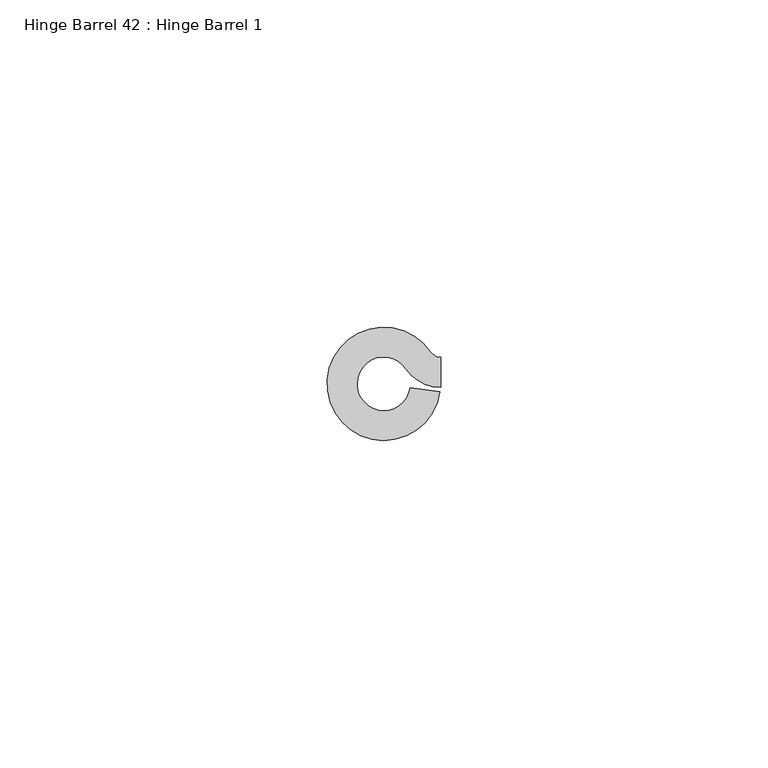
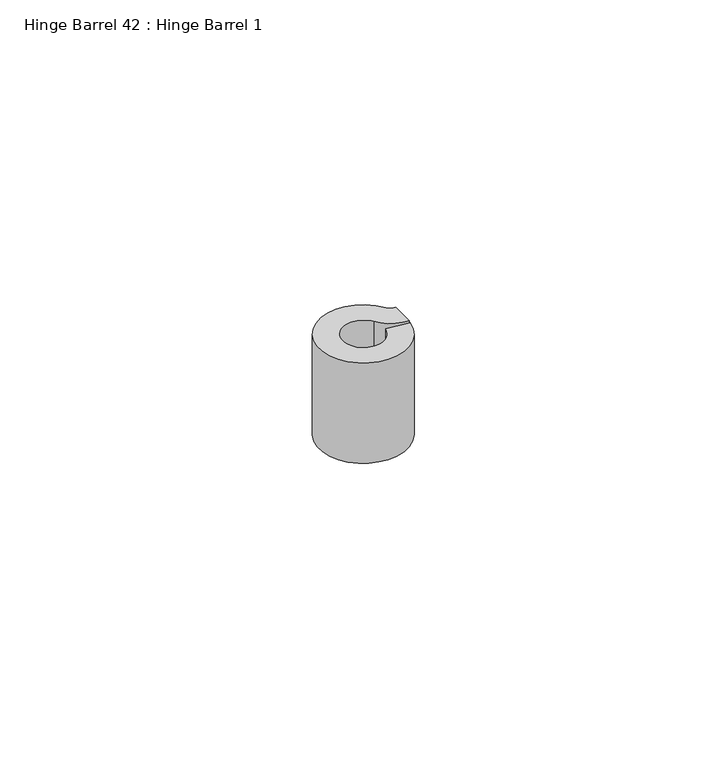
"""IFC4 building model written with IfcOpenShell, lengths in millimetres: proxy geometry, Hinge Barrel 42 : Hinge Barrel 1."""

from ifc_helpers import new_model, si_unit, point, frame, frame_2d, origin, place, context, project, spatial, polyline, circle_curve, trimmed, segment, composite_curve, outline, extrude, source, transform, mapped, element, save


def hinge_barrel_42_hinge_barrel_1_1e33f8db(model_context):
    return source(origin(), model_context, "Body", "SweptSolid", [
        extrude(outline(composite_curve([segment(trimmed(circle_curve(frame_2d((587319.1320739, -534100.7049841)), 4.0894), [point((587322.5194669, -534098.4139665))], [point((587323.1821338, -534101.2708529))], True, "CARTESIAN"), True, "CONTINUOUS"), segment(polyline([(587323.1821338, -534101.2708529), (587327.7022899, -534101.9024028)]), True, "CONTINUOUS"), segment(trimmed(circle_curve(frame_2d((587319.1320739, -534100.7049841)), 8.6534625), [point((587327.7022899, -534101.9024028))], [point((587326.3000393, -534095.8570273))], False, "CARTESIAN"), True, "CONTINUOUS"), segment(trimmed(circle_curve(frame_2d((587327.8245257, -534094.8259615)), 1.8404226), [point((587326.3000393, -534095.8570273))], [point((587327.8245257, -534096.6663841))], True, "CARTESIAN"), True, "CONTINUOUS"), segment(polyline([(587327.8245257, -534096.6663841), (587327.8245257, -534101.2304466)]), True, "CONTINUOUS"), segment(trimmed(circle_curve(frame_2d((587327.8245257, -534094.8259615)), 6.4044851), [point((587327.8245257, -534101.2304466))], [point((587322.5194669, -534098.4139665))], False, "CARTESIAN"), True, "CONTINUOUS")], self_intersect=False)), frame((0.0, 0.0, 438.15), z_axis=(0.0, 0.0, 1.0), x_axis=(1.0, 0.0, 0.0)), (0.0, 0.0, 1.0), 20.8359375),
    ])


if __name__ == "__main__":
    model = new_model("IFC4")
    model_context = context("Model", 3, world=origin())
    ifc_project = project(units=[si_unit("LENGTHUNIT", "METRE", prefix="MILLI")], contexts=[model_context])
    site = spatial("IfcSite", under=ifc_project)
    building = spatial("IfcBuilding", under=site)
    placement = place(None, origin())
    hinge_barrel_42_hinge_barrel_1_shape = hinge_barrel_42_hinge_barrel_1_1e33f8db(model_context)
    element("IfcBuildingElementProxy", 1, Name="Hinge Barrel 42 : Hinge Barrel 1", ObjectType="Hinge Barrel 42 : Hinge Barrel 1", at=placement, inside=building, context=model_context, shape_type="MappedRepresentation", body=[
        mapped(hinge_barrel_42_hinge_barrel_1_shape, transform((0.0, 0.0, 0.0), x_axis=(1.0, 0.0, 0.0), y_axis=(0.0, 1.0, 0.0), z_axis=(0.0, 0.0, 1.0))),
    ])
    save(model, "model.ifc")

# Revit data of these elements
# Element 1 (IfcBuildingElementProxy, "Hinge Barrel 42 : Hinge Barrel 1")
#   Materials on its faces: "6\"X6\" WELD-ON STL BUTT HINGE"
# Materials
#   "6\"X6\" WELD-ON STL BUTT HINGE": class "Metal", colour RGB 189 187 185, transparency 0, Description = "Carbon steel", Cost = 0
